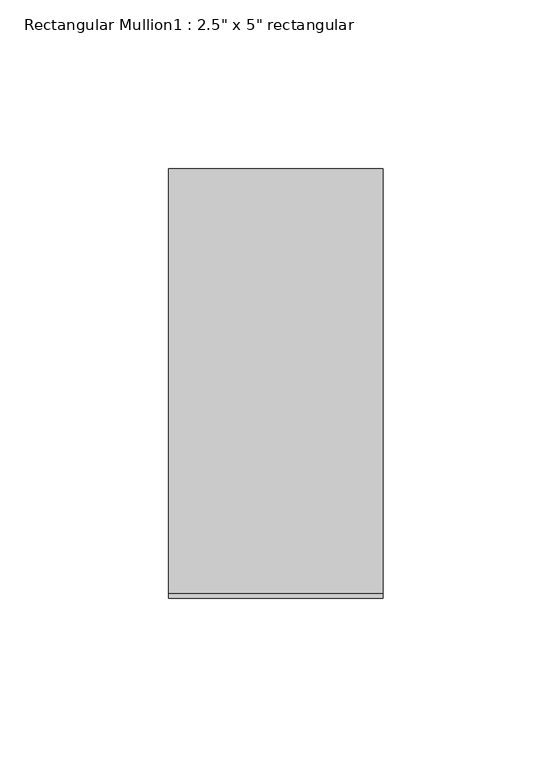
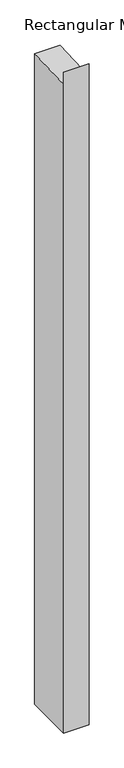
"""IFC4 building model written with IfcOpenShell, lengths in millimetres: member geometry."""

from ifc_helpers import new_model, si_unit, frame, origin, place, context, project, spatial, polyline, outline, extrude, source, transform, mapped, element, save


def member_0a0eb772(model_context):
    return source(origin(), model_context, "Body", "SweptSolid", [
        extrude(outline(polyline([(-63.5, 30.4748075), (-62.1741259, -2.5237591), (63.5, 2.5257955), (63.5, -1733.5500228), (-63.5, -1733.5500228), (-63.5, 30.4748075)])), frame((-63.5, 0.0, 0.0), z_axis=(1.0, 0.0, 0.0), x_axis=(0.0, 1.0, 0.0)), (0.0, 0.0, 1.0), 63.5),
    ])


if __name__ == "__main__":
    model = new_model("IFC4")
    model_context = context("Model", 3, world=origin())
    ifc_project = project(units=[si_unit("LENGTHUNIT", "METRE", prefix="MILLI")], contexts=[model_context])
    site = spatial("IfcSite", under=ifc_project)
    building = spatial("IfcBuilding", under=site)
    placement = place(None, origin())
    member_shape = member_0a0eb772(model_context)
    element("IfcMember", 1, ObjectType="Rectangular Mullion1 : 2.5\" x 5\" rectangular", at=placement, inside=building, context=model_context, shape_type="MappedRepresentation", body=[
        mapped(member_shape, transform((0.0, 0.0, 0.0), x_axis=(1.0, 0.0, 0.0), y_axis=(0.0, 1.0, 0.0), z_axis=(0.0, 0.0, 1.0))),
    ])
    save(model, "model.ifc")

# Revit data of these elements
# Type "Rectangular Mullion1 : 2.5\" x 5\" rectangular"
#   built-in parameter 1007304 = 0.416667 (stored number, unit not read)
#   built-in parameter 1007301 = 0.104167 (stored number, unit not read)
#   built-in parameter 1007300 = 0.104167 (stored number, unit not read)
# Element 1 (IfcMember, "Rectangular Mullion1 : 2.5\" x 5\" rectangular")
#   Materials on its faces: "support-frame"
# Materials
#   "support-frame": class "Unassigned", colour RGB 233 233 233, transparency 0, Cost = 0
